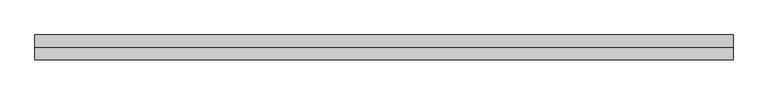
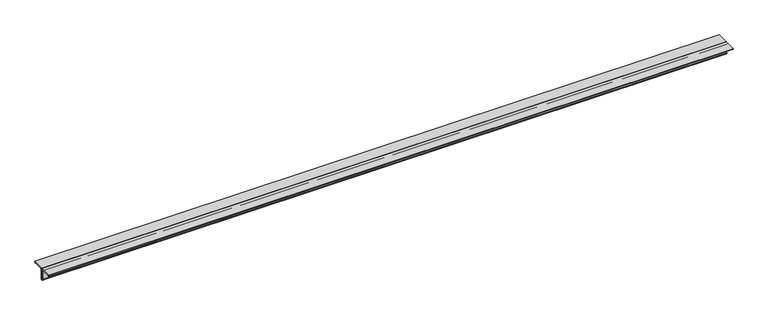
"""IFC4 building model written with IfcOpenShell, lengths in millimetres: member geometry, Steel Framing_2Ls_KS : H_SB_AR_S02_2Ls-100x100x10_VBR1."""

from ifc_helpers import new_model, si_unit, point, frame, frame_2d, origin, place, context, project, spatial, polyline, circle_curve, trimmed, segment, composite_curve, outline, extrude, source, transform, mapped, element, save


def member_53cc3ac8(model_context):
    return source(origin(), model_context, "Body", "SweptSolid", [
        extrude(outline(composite_curve([segment(polyline([(0.0, 28.2), (100.0, 28.2)]), True, "CONTINUOUS"), segment(trimmed(circle_curve(frame_2d((90.0, 28.2)), 10.0), [point((100.0, 28.2))], [point((90.0, 18.2))], False, "CARTESIAN"), True, "CONTINUOUS"), segment(polyline([(90.0, 18.2), (20.0, 18.2)]), True, "CONTINUOUS"), segment(trimmed(circle_curve(frame_2d((20.0, 8.2)), 10.0), [point((20.0, 18.2))], [point((10.0, 8.2))], True, "CARTESIAN"), True, "CONTINUOUS"), segment(polyline([(10.0, 8.2), (10.0, -61.8)]), True, "CONTINUOUS"), segment(trimmed(circle_curve(frame_2d((0.0, -61.8)), 10.0), [point((10.0, -61.8))], [point((0.0, -71.8))], False, "CARTESIAN"), True, "CONTINUOUS"), segment(polyline([(0.0, -71.8), (0.0, 28.2)]), True, "CONTINUOUS")], self_intersect=False)), frame((-2916.9883392, 0.0, 0.0), z_axis=(1.0, 0.0, 0.0), x_axis=(0.0, 1.0, 0.0)), (0.0, 0.0, 1.0), 5637.64946),
        extrude(outline(composite_curve([segment(polyline([(0.0, 28.2), (0.0, -71.8)]), True, "CONTINUOUS"), segment(trimmed(circle_curve(frame_2d((0.0, -61.8)), 10.0), [point((0.0, -71.8))], [point((-10.0, -61.8))], False, "CARTESIAN"), True, "CONTINUOUS"), segment(polyline([(-10.0, -61.8), (-10.0, 8.2)]), True, "CONTINUOUS"), segment(trimmed(circle_curve(frame_2d((-20.0, 8.2)), 10.0), [point((-10.0, 8.2))], [point((-20.0, 18.2))], True, "CARTESIAN"), True, "CONTINUOUS"), segment(polyline([(-20.0, 18.2), (-90.0, 18.2)]), True, "CONTINUOUS"), segment(trimmed(circle_curve(frame_2d((-90.0, 28.2)), 10.0), [point((-90.0, 18.2))], [point((-100.0, 28.2))], False, "CARTESIAN"), True, "CONTINUOUS"), segment(polyline([(-100.0, 28.2), (0.0, 28.2)]), True, "CONTINUOUS")], self_intersect=False)), frame((-2916.9883392, 0.0, 0.0), z_axis=(1.0, 0.0, 0.0), x_axis=(0.0, 1.0, 0.0)), (0.0, 0.0, 1.0), 5637.64946),
    ])


if __name__ == "__main__":
    model = new_model("IFC4")
    model_context = context("Model", 3, world=origin())
    ifc_project = project(units=[si_unit("LENGTHUNIT", "METRE", prefix="MILLI")], contexts=[model_context])
    site = spatial("IfcSite", under=ifc_project)
    building = spatial("IfcBuilding", under=site)
    placement = place(None, origin())
    member_shape = member_53cc3ac8(model_context)
    element("IfcMember", 1, ObjectType="Steel Framing_2Ls_KS : H_SB_AR_S02_2Ls-100x100x10_VBR1", at=placement, inside=building, context=model_context, shape_type="MappedRepresentation", body=[
        mapped(member_shape, transform((0.0, 0.0, 0.0), x_axis=(1.0, 0.0, 0.0), y_axis=(0.0, 1.0, 0.0), z_axis=(0.0, 0.0, 1.0))),
    ])
    save(model, "model.ifc")

# Revit data of these elements
# Type "Steel Framing_2Ls_KS : H_SB_AR_S02_2Ls-100x100x10_VBR1"
#   Type Comments = "MAIN"
#   Type Mark = "VBR1"
#   H_SectionID = "2Ls-100x100x10"
#   Assembly Code = "B10"
#   Legs = "LLBB"
#   H_Ratio for Additional Steel Plate = 0.2
#   W = 0
#   Perimeter = 0.80 m²/m
#   Nominal Weight = 29.80 kgf/m
#   Length [instance default] = 1524 mm
#   Space = 0 mm
#   b = 100 mm
#   d = 100 mm
#   t = 10 mm
#   y = 28.2 mm
#   A = 0.0038 m²
#   Structural Material [instance default] = Steel, 45-345
# Element 1 (IfcMember, "Steel Framing_2Ls_KS : H_SB_AR_S02_2Ls-100x100x10_VBR1")
#   Materials on its faces: "Steel, 45-345"
# Materials
#   "Steel, 45-345": class "Metal", colour RGB 189 187 185, transparency 0, Description = "Steel 345 MPa", Cost = 0
